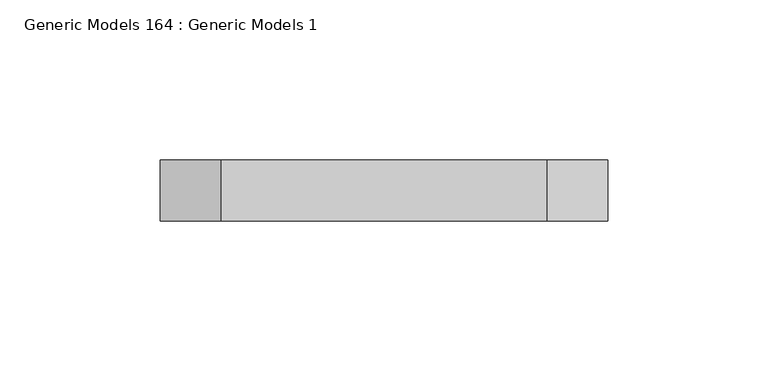
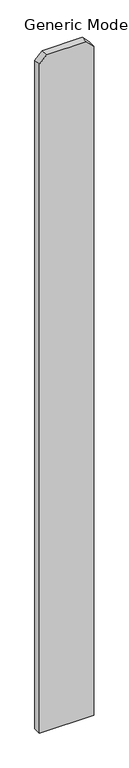
"""IFC4 building model written with IfcOpenShell, lengths in millimetres: proxy geometry, Generic Models 164 : Generic Models 1."""

from ifc_helpers import new_model, si_unit, frame, origin, place, context, project, spatial, polyline, outline, extrude, source, transform, mapped, element, save


def generic_models_164_generic_models_1_c75473e5(model_context):
    return source(origin(), model_context, "Body", "SweptSolid", [
        extrude(outline(polyline([(76.2, 54989.4125), (1885.95, 54989.4125), (1905.0, 54970.3625), (1905.0, 54868.7625), (1885.95, 54849.7125), (76.2, 54849.7125), (76.2, 54989.4125)])), frame((0.0, 547.6875, 0.0), z_axis=(0.0, 1.0, 0.0), x_axis=(0.0, 0.0, 1.0)), (0.0, 0.0, 1.0), 19.05),
    ])


if __name__ == "__main__":
    model = new_model("IFC4")
    model_context = context("Model", 3, world=origin())
    ifc_project = project(units=[si_unit("LENGTHUNIT", "METRE", prefix="MILLI")], contexts=[model_context])
    site = spatial("IfcSite", under=ifc_project)
    building = spatial("IfcBuilding", under=site)
    placement = place(None, origin())
    generic_models_164_generic_models_1_shape = generic_models_164_generic_models_1_c75473e5(model_context)
    element("IfcBuildingElementProxy", 1, Name="Generic Models 164 : Generic Models 1", ObjectType="Generic Models 164 : Generic Models 1", at=placement, inside=building, context=model_context, shape_type="MappedRepresentation", body=[
        mapped(generic_models_164_generic_models_1_shape, transform((0.0, 0.0, 0.0), x_axis=(1.0, 0.0, 0.0), y_axis=(0.0, 1.0, 0.0), z_axis=(0.0, 0.0, 1.0))),
    ])
    save(model, "model.ifc")

# Revit data of these elements
# Element 1 (IfcBuildingElementProxy, "Generic Models 164 : Generic Models 1")
#   Materials on its faces: "VERTICAL 1X6 CEDAR PLANKS W/ CLEAR WOOD SEALER"
# Materials
#   "VERTICAL 1X6 CEDAR PLANKS W/ CLEAR WOOD SEALER": class "Wood", colour RGB 234 198 147, transparency 0, Description = "Pinus Echinata", Cost = 0
